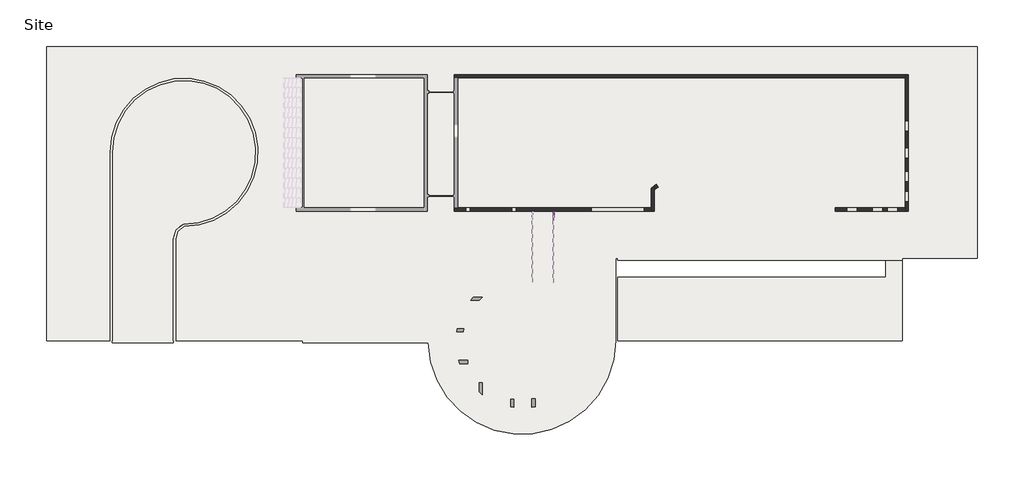
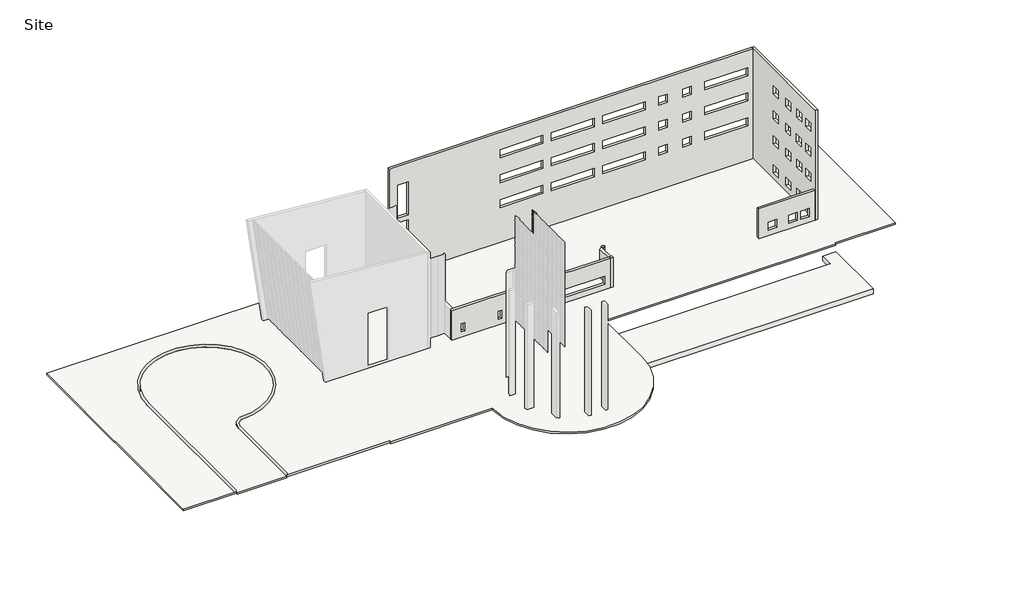
# One storey, part 4 of 4: 17 members, 6 walls, 3 slabs, 1 plate.
"""IFC4 building model written with IfcOpenShell, lengths in millimetres."""

import ifcopenshell
import ifcopenshell.guid

model = None  # the IFC model being written
_history = None  # IfcOwnerHistory: only IFC2X3 demands one
_inside = {}  # id of a spatial element -> (the spatial element, [elements in it])
_under = {}  # id of a project, library or spatial element -> (it, [spatial elements below it])
_declared = {}  # id of a project -> (the project, [libraries it declares])
_typed = {}  # id of a type object -> (the type object, [elements of that type])
_made_of = {}  # id of a material, layer set ... -> (it, [elements and type objects made of it])


def new_model(schema):
    """Start an empty IFC model of exactly this schema.

    Asked for "IFC4X3", IfcOpenShell would pick the latest addendum, in which some entities
    have other attributes; the version numbers below select the first issue.
    IFC2X3 requires an IfcOwnerHistory on every rooted entity: one is made here for all.
    """
    global model, _history
    if schema == "IFC4X3":
        model = ifcopenshell.file(schema_version=(4, 3, 0, 0))
    else:
        model = ifcopenshell.file(schema=schema)
    _inside.clear()
    _under.clear()
    _declared.clear()
    _typed.clear()
    _made_of.clear()
    _history = None
    if model.schema == "IFC2X3":
        org = make("IfcOrganization", Name="unknown")
        user = make(
            "IfcPersonAndOrganization",
            ThePerson=make("IfcPerson", FamilyName="unknown"),
            TheOrganization=org,
        )
        app = make(
            "IfcApplication",
            ApplicationDeveloper=org,
            Version="unknown",
            ApplicationFullName="unknown",
            ApplicationIdentifier="unknown",
        )
        _history = make(
            "IfcOwnerHistory",
            OwningUser=user,
            OwningApplication=app,
            ChangeAction="ADDED",
            CreationDate=0,
        )
    return model


def make(cls, **values):
    """One entity of the class cls with the attributes given. An attribute that is None is left unset."""
    return model.create_entity(
        cls, **{name: value for name, value in values.items() if value is not None}
    )


def rooted(cls, **values):
    """An entity with a GlobalId (a new one), such as an element, a storey or a relation."""
    return make(cls, GlobalId=ifcopenshell.guid.new(), OwnerHistory=_history, **values)


def si_unit(unit_type, name, prefix=None):
    """IfcSIUnit, for example si_unit("LENGTHUNIT", "METRE", prefix="MILLI")."""
    return make("IfcSIUnit", UnitType=unit_type, Prefix=prefix, Name=name)


def assignment(units):
    """IfcUnitAssignment: the units of a project."""
    return None if units is None else make("IfcUnitAssignment", Units=units)


def point(xyz):
    """IfcCartesianPoint."""
    return None if xyz is None else make("IfcCartesianPoint", Coordinates=xyz)


def direction(xyz):
    """IfcDirection."""
    return None if xyz is None else make("IfcDirection", DirectionRatios=xyz)


def frame(location, z_axis=None, x_axis=None):
    """IfcAxis2Placement3D, a coordinate frame: its origin and axes. An axis left out is left unset."""
    return make(
        "IfcAxis2Placement3D",
        Location=point(location),
        Axis=direction(z_axis),
        RefDirection=direction(x_axis),
    )


def frame_2d(location, x_axis=None):
    """IfcAxis2Placement2D, a coordinate frame in the plane: its origin and x axis."""
    return make(
        "IfcAxis2Placement2D", Location=point(location), RefDirection=direction(x_axis)
    )


def origin():
    """The frame at (0, 0, 0) with its axes left unset."""
    return frame((0.0, 0.0, 0.0))


def origin_with_axes():
    """The frame at (0, 0, 0) with the z axis (0, 0, 1) and the x axis (1, 0, 0) written out."""
    return frame((0.0, 0.0, 0.0), z_axis=(0.0, 0.0, 1.0), x_axis=(1.0, 0.0, 0.0))


def place(relative_to, where):
    """IfcLocalPlacement: puts the frame where relative to a parent placement (None: the world)."""
    return make(
        "IfcLocalPlacement", PlacementRelTo=relative_to, RelativePlacement=where
    )


def context(
    kind, dimensions, precision=None, world=None, true_north=None, identifier=None
):
    """IfcGeometricRepresentationContext, for example the 3D "Model" context."""
    return make(
        "IfcGeometricRepresentationContext",
        ContextIdentifier=identifier,
        ContextType=kind,
        CoordinateSpaceDimension=dimensions,
        Precision=precision,
        WorldCoordinateSystem=world,
        TrueNorth=true_north,
    )


def project(units=None, contexts=None):
    """IfcProject with its units and contexts."""
    return rooted(
        "IfcProject",
        Name="project",
        RepresentationContexts=contexts,
        UnitsInContext=assignment(units),
    )


def spatial(cls, under=None, at=None, **own):
    """A site, building, storey or space (cls), placed at a placement, below another one or the project."""
    s = rooted(cls, ObjectPlacement=at, **own)
    if under is not None:
        _under.setdefault(under.id(), (under, []))[1].append(s)
    return s


def polyline(points):
    """IfcPolyline through the points."""
    return make("IfcPolyline", Points=[point(p) for p in points])


def circle_curve(where, radius):
    """IfcCircle in the frame where."""
    return make("IfcCircle", Position=where, Radius=radius)


def trimmed(basis, trim1, trim2, sense, master):
    """IfcTrimmedCurve: the piece of a basis curve between two trims."""
    return make(
        "IfcTrimmedCurve",
        BasisCurve=basis,
        Trim1=trim1,
        Trim2=trim2,
        SenseAgreement=sense,
        MasterRepresentation=master,
    )


def segment(curve, same_sense, transition):
    """IfcCompositeCurveSegment."""
    return make(
        "IfcCompositeCurveSegment",
        Transition=transition,
        SameSense=same_sense,
        ParentCurve=curve,
    )


def composite_curve(segments, self_intersect=None):
    """IfcCompositeCurve: segments joined end to end."""
    return make("IfcCompositeCurve", Segments=segments, SelfIntersect=self_intersect)


def outline(outer, holes=None, kind="AREA"):
    """IfcArbitraryClosedProfileDef: a profile drawn as a closed curve; with holes, ...WithVoids."""
    if holes is None:
        return make("IfcArbitraryClosedProfileDef", ProfileType=kind, OuterCurve=outer)
    return make(
        "IfcArbitraryProfileDefWithVoids",
        ProfileType=kind,
        OuterCurve=outer,
        InnerCurves=holes,
    )


def extrude(swept, where, along, depth):
    """IfcExtrudedAreaSolid: the profile swept, set in the frame where, extruded along a direction by depth."""
    return make(
        "IfcExtrudedAreaSolid",
        SweptArea=swept,
        Position=where,
        ExtrudedDirection=direction(along),
        Depth=depth,
    )


def faces_of(points, faces, orient=None, outer=None):
    """IfcFace entities. A face is a list of loops; a loop is a list of indices into points, from 0.

    orient and outer hold one flag for each loop. By default every Orientation is true, the
    first loop of a face is its IfcFaceOuterBound and the others are IfcFaceBound.
    """
    made = []
    for i, loops in enumerate(faces):
        bounds = []
        for j, loop in enumerate(loops):
            is_outer = j == 0 if outer is None else outer[i][j]
            bounds.append(
                make(
                    "IfcFaceOuterBound" if is_outer else "IfcFaceBound",
                    Bound=make("IfcPolyLoop", Polygon=[points[k] for k in loop]),
                    Orientation=True if orient is None else orient[i][j],
                )
            )
        made.append(make("IfcFace", Bounds=bounds))
    return made


def faceted_brep(points, faces, orient=None, outer=None, voids=None):
    """IfcFacetedBrep: a solid bounded by flat faces; with voids (closed shells), ...WithVoids."""
    shared = [point(p) for p in points]
    hull = make("IfcClosedShell", CfsFaces=faces_of(shared, faces, orient, outer))
    if voids is None:
        return make("IfcFacetedBrep", Outer=hull)
    return make(
        "IfcFacetedBrepWithVoids",
        Outer=hull,
        Voids=[
            make(cls, CfsFaces=faces_of(shared, fs, o, b)) for cls, fs, o, b in voids
        ],
    )


def shape(context_of_items, identifier, shape_type, items):
    """IfcShapeRepresentation: the items that make up one representation, for example the "Body"."""
    return make(
        "IfcShapeRepresentation",
        ContextOfItems=context_of_items,
        RepresentationIdentifier=identifier,
        RepresentationType=shape_type,
        Items=items,
    )


def source(mapping_origin, context_of_items, identifier, shape_type, items):
    """IfcRepresentationMap: a shape defined once, which mapped items show again and again."""
    return make(
        "IfcRepresentationMap",
        MappingOrigin=mapping_origin,
        MappedRepresentation=shape(context_of_items, identifier, shape_type, items),
    )


def transform(
    local_origin,
    x_axis=None,
    y_axis=None,
    z_axis=None,
    scale=None,
    scale2=None,
    scale3=None,
    uniform=True,
):
    """IfcCartesianTransformationOperator3D, or its non-uniform kind. x_axis, y_axis, z_axis: its Axis1, 2, 3."""
    if uniform:
        return make(
            "IfcCartesianTransformationOperator3D",
            Axis1=direction(x_axis),
            Axis2=direction(y_axis),
            LocalOrigin=point(local_origin),
            Scale=scale,
            Axis3=direction(z_axis),
        )
    return make(
        "IfcCartesianTransformationOperator3DnonUniform",
        Axis1=direction(x_axis),
        Axis2=direction(y_axis),
        LocalOrigin=point(local_origin),
        Scale=scale,
        Axis3=direction(z_axis),
        Scale2=scale2,
        Scale3=scale3,
    )


def mapped(mapping_source, mapping_target):
    """IfcMappedItem: shows the shape of a source again, moved by a transform."""
    return make(
        "IfcMappedItem", MappingSource=mapping_source, MappingTarget=mapping_target
    )


def made_of(thing, what):
    """Note that an element or type object is made of a material, layer set ...; save() writes the relation."""
    if what is not None:
        _made_of.setdefault(what.id(), (what, []))[1].append(thing)
    return thing


def element(
    cls,
    number,
    at=None,
    inside=None,
    cuts=None,
    type_object=None,
    material=None,
    context=None,
    identifier="Body",
    shape_type=None,
    held_by="IfcProductDefinitionShape",
    body=None,
    shapes=None,
    **own,
):
    """One element of the class cls, such as IfcWall. Its Tag is "e" and its number.

    at: its placement. inside: the storey or other place that contains it. cuts: it is an
    opening in that element (IfcRelVoidsElement). A single representation is given by context,
    identifier, shape_type and body (its items); several are given by shapes. held_by: the class
    of the entity that holds the representations. save() writes the other relations.
    """
    e = rooted(cls, Tag="e%d" % number, ObjectPlacement=at, **own)
    if body is not None:
        shapes = [shape(context, identifier, shape_type, body)]
    if shapes is not None:
        e.Representation = make(held_by, Representations=shapes)
    if inside is not None:
        _inside.setdefault(inside.id(), (inside, []))[1].append(e)
    if cuts is not None:
        rooted(
            "IfcRelVoidsElement", RelatingBuildingElement=cuts, RelatedOpeningElement=e
        )
    if type_object is not None:
        _typed.setdefault(type_object.id(), (type_object, []))[1].append(e)
    return made_of(e, material)


def aggregate(whole, parts):
    """IfcRelAggregates: a whole, such as a stair, and the parts it consists of."""
    return rooted("IfcRelAggregates", RelatingObject=whole, RelatedObjects=parts)


def save(model, path):
    """Write the relations noted so far, then the file.

    IfcRelAggregates (storeys below a building ...), IfcRelContainedInSpatialStructure (elements
    in a storey), IfcRelDefinesByType, IfcRelAssociatesMaterial and IfcRelDeclares: one each for
    every whole, place, type object, material and project.
    """
    for whole, parts in _under.values():
        aggregate(whole, parts)
    for where, things in _inside.values():
        rooted(
            "IfcRelContainedInSpatialStructure",
            RelatedElements=things,
            RelatingStructure=where,
        )
    for kind, things in _typed.values():
        rooted("IfcRelDefinesByType", RelatedObjects=things, RelatingType=kind)
    for what, things in _made_of.values():
        rooted("IfcRelAssociatesMaterial", RelatedObjects=things, RelatingMaterial=what)
    for by, libraries in _declared.values():
        rooted("IfcRelDeclares", RelatingContext=by, RelatedDefinitions=libraries)
    model.write(path)


def plane_surface(at):
    """IfcPlane: the flat surface through the origin of the frame at, square to its z axis."""
    return make("IfcPlane", Position=at)


def cylinder_surface(at, radius):
    """IfcCylindricalSurface: all points at the distance radius from the z axis of the frame at."""
    return make("IfcCylindricalSurface", Position=at, Radius=radius)


def revolved_surface(curve, axis_point, axis_direction):
    """IfcSurfaceOfRevolution: the curve turned about the line through axis_point along axis_direction."""
    return make(
        "IfcSurfaceOfRevolution",
        SweptCurve=make("IfcArbitraryOpenProfileDef", ProfileType="CURVE", Curve=curve),
        AxisPosition=make("IfcAxis1Placement", Location=point(axis_point), Axis=direction(axis_direction)),
    )


def advanced_brep(points, edges, surfaces, faces):
    """IfcAdvancedBrep: a solid bounded by faces that lie on surfaces and meet in shared edges.

    An edge is (start, end): straight between two places in points (the first is 0);
    or (start, end, curve); or (start, end, curve, False) where it runs against its curve.
    A face is (place in surfaces, loops), or (place, loops, False) where it looks against
    its surface's normal. A loop lists edges by number (the first is 1), with a minus sign
    where the edge is run from its end to its start. The first loop is the outer one.
    """
    corners = [point(p) for p in points]
    vertices = [make("IfcVertexPoint", VertexGeometry=c) for c in corners]
    made = []
    for start, end, *more in edges:
        made.append(
            make(
                "IfcEdgeCurve",
                EdgeStart=vertices[start],
                EdgeEnd=vertices[end],
                EdgeGeometry=more[0] if more else make("IfcPolyline", Points=[corners[start], corners[end]]),
                SameSense=more[1] if len(more) > 1 else True,
            )
        )
    hull = []
    for where, loops, *sense in faces:
        bounds = []
        for j, loop in enumerate(loops):
            ring = [make("IfcOrientedEdge", EdgeElement=made[abs(k) - 1], Orientation=k > 0) for k in loop]
            bounds.append(
                make(
                    "IfcFaceOuterBound" if j == 0 else "IfcFaceBound",
                    Bound=make("IfcEdgeLoop", EdgeList=ring),
                    Orientation=True,
                )
            )
        hull.append(make("IfcAdvancedFace", Bounds=bounds, FaceSurface=surfaces[where], SameSense=sense[0] if sense else True))
    return make("IfcAdvancedBrep", Outer=make("IfcClosedShell", CfsFaces=hull))


def member_5d07894b(model_context):
    return source(origin(), model_context, "Body", "SweptSolid", [
        extrude(outline(polyline([(31.75, 63.5), (31.75, -63.5), (-31.75, -63.5), (-31.75, 63.5), (31.75, 63.5)])), frame((0.0, 0.0, -4629.15), z_axis=(0.0, 0.0, 1.0), x_axis=(1.0, 0.0, 0.0)), (0.0, 0.0, 1.0), 4629.15),
    ])


def member_3ba9e939(model_context):
    return source(origin(), model_context, "Body", "SweptSolid", [
        extrude(outline(polyline([(31.75, 63.5), (31.75, -63.5), (-31.75, -63.5), (-31.75, 63.5), (31.75, 63.5)])), frame((0.0, 0.0, -3746.5), z_axis=(0.0, 0.0, 1.0), x_axis=(1.0, 0.0, 0.0)), (0.0, 0.0, 1.0), 3746.5),
    ])


def member_ad567e07(model_context):
    return source(origin(), model_context, "Body", "SweptSolid", [
        extrude(outline(polyline([(31.75, 63.5), (31.75, -63.5), (-31.75, -63.5), (-31.75, 63.5), (31.75, 63.5)])), frame((0.0, 0.0, -819.15), z_axis=(0.0, 0.0, 1.0), x_axis=(1.0, 0.0, 0.0)), (0.0, 0.0, 1.0), 819.15),
    ])


def member_7db1855a(model_context):
    return source(origin(), model_context, "Body", "SweptSolid", [
        extrude(outline(polyline([(31.75, 63.5), (31.75, -63.5), (-31.75, -63.5), (-31.75, 63.5), (31.75, 63.5)])), frame((0.0, 0.0, -850.9), z_axis=(0.0, 0.0, 1.0), x_axis=(1.0, 0.0, 0.0)), (0.0, 0.0, 1.0), 850.9),
    ])


def member_ffd4c858(model_context):
    return source(origin(), model_context, "Body", "SweptSolid", [
        extrude(outline(polyline([(31.75, 63.5), (31.75, -63.5), (-31.75, -63.5), (-31.75, 63.5), (31.75, 63.5)])), frame((0.0, 0.0, -457.2), z_axis=(0.0, 0.0, 1.0), x_axis=(1.0, 0.0, 0.0)), (0.0, 0.0, 1.0), 457.2),
    ])


def member_15823cb3(model_context):
    return source(origin(), model_context, "Body", "SweptSolid", [
        extrude(outline(polyline([(0.0, 63.5), (0.0, -63.5), (-63.5, -63.5), (-63.5, 63.5), (0.0, 63.5)])), frame((0.0, 0.0, -457.2), z_axis=(0.0, 0.0, 1.0), x_axis=(1.0, 0.0, 0.0)), (0.0, 0.0, 1.0), 457.2),
    ])


def member_e9605c56(model_context):
    return source(origin(), model_context, "Body", "SweptSolid", [
        extrude(outline(polyline([(0.0, 63.5), (0.0, -63.5), (-63.5, -63.5), (-63.5, 63.5), (0.0, 63.5)])), frame((0.0, 0.0, -825.5), z_axis=(0.0, 0.0, 1.0), x_axis=(1.0, 0.0, 0.0)), (0.0, 0.0, 1.0), 825.5),
    ])


def system_panel_glazed_cc98a0ec(model_context):
    return source(origin(), model_context, "Body", "SweptSolid", [
        extrude(outline(polyline([(180.975, 19.05), (-180.975, 19.05), (-180.975, 44.45), (180.975, 44.45), (180.975, 19.05)])), origin_with_axes(), (0.0, 0.0, 1.0), 819.15),
    ])


model = new_model("IFC4")

# Units and contexts
model_context = context("Model", 3, world=origin())
ifc_project = project(units=[si_unit("LENGTHUNIT", "METRE", prefix="MILLI")], contexts=[model_context])

# Site, building, storey
site = spatial("IfcSite", under=ifc_project)
building = spatial("IfcBuilding", under=site)
storey = spatial("IfcBuildingStorey", under=building, Name="Site", Elevation=-152.4)

# Members
placement = place(None, origin())
member_shape = member_5d07894b(model_context)
element("IfcMember", 1, ObjectType="Rectangular Mullion1 : 2.5\" x 5\" rectangular", at=placement, inside=storey, context=model_context, shape_type="MappedRepresentation", body=[
    mapped(member_shape, transform((10878.8276119, 37629.311889, -88.9), x_axis=(0.0, 1.0, 0.0), y_axis=(1.0, 0.0, 0.0), z_axis=(0.0, 0.0, -1.0))),
])
member_2_shape = member_3ba9e939(model_context)
element("IfcMember", 2, ObjectType="Rectangular Mullion1 : 2.5\" x 5\" rectangular", at=placement, inside=storey, context=model_context, shape_type="MappedRepresentation", body=[
    mapped(member_2_shape, transform((10878.8276119, 37629.311889, 5518.15), x_axis=(0.0, 1.0, 0.0), y_axis=(1.0, 0.0, 0.0), z_axis=(0.0, 0.0, -1.0))),
])
element("IfcMember", 3, ObjectType="Rectangular Mullion1 : 2.5\" x 5\" rectangular", at=placement, inside=storey, context=model_context, shape_type="MappedRepresentation", body=[
    mapped(member_2_shape, transform((10878.8276119, 37629.311889, 10242.55), x_axis=(0.0, 1.0, 0.0), y_axis=(1.0, 0.0, 0.0), z_axis=(0.0, 0.0, -1.0))),
])
element("IfcMember", 4, ObjectType="Rectangular Mullion1 : 2.5\" x 5\" rectangular", at=placement, inside=storey, context=model_context, shape_type="MappedRepresentation", body=[
    mapped(member_2_shape, transform((10878.8276119, 37629.311889, 14966.95), x_axis=(0.0, 1.0, 0.0), y_axis=(1.0, 0.0, 0.0), z_axis=(0.0, 0.0, -1.0))),
])
member_3_shape = member_ad567e07(model_context)
element("IfcMember", 5, ObjectType="Rectangular Mullion1 : 2.5\" x 5\" rectangular", at=placement, inside=storey, context=model_context, shape_type="MappedRepresentation", body=[
    mapped(member_3_shape, transform((10878.8276119, 37629.311889, 18776.95), x_axis=(0.0, 1.0, 0.0), y_axis=(1.0, 0.0, 0.0), z_axis=(0.0, 0.0, -1.0))),
])
member_4_shape = member_7db1855a(model_context)
element("IfcMember", 6, ObjectType="Rectangular Mullion1 : 2.5\" x 5\" rectangular", at=placement, inside=storey, context=model_context, shape_type="MappedRepresentation", body=[
    mapped(member_4_shape, transform((10878.8276119, 37629.311889, 14052.55), x_axis=(0.0, 1.0, 0.0), y_axis=(1.0, 0.0, 0.0), z_axis=(0.0, 0.0, -1.0))),
])
element("IfcMember", 7, ObjectType="Rectangular Mullion1 : 2.5\" x 5\" rectangular", at=placement, inside=storey, context=model_context, shape_type="MappedRepresentation", body=[
    mapped(member_4_shape, transform((10878.8276119, 37629.311889, 4603.75), x_axis=(0.0, 1.0, 0.0), y_axis=(1.0, 0.0, 0.0), z_axis=(0.0, 0.0, -1.0))),
])
element("IfcMember", 8, ObjectType="Rectangular Mullion1 : 2.5\" x 5\" rectangular", at=placement, inside=storey, context=model_context, shape_type="MappedRepresentation", body=[
    mapped(member_4_shape, transform((10878.8276119, 37629.311889, 9328.15), x_axis=(0.0, 1.0, 0.0), y_axis=(1.0, 0.0, 0.0), z_axis=(0.0, 0.0, -1.0))),
])
member_5_shape = member_ffd4c858(model_context)
element("IfcMember", 9, ObjectType="Rectangular Mullion1 : 2.5\" x 5\" rectangular", at=placement, inside=storey, context=model_context, shape_type="MappedRepresentation", body=[
    mapped(member_5_shape, transform((10878.8276119, 38086.511889, 14935.2), x_axis=(0.0, 0.0, 1.0), y_axis=(1.0, 0.0, 0.0), z_axis=(0.0, 1.0, 0.0))),
])
element("IfcMember", 10, ObjectType="Rectangular Mullion1 : 2.5\" x 5\" rectangular", at=placement, inside=storey, context=model_context, shape_type="MappedRepresentation", body=[
    mapped(member_5_shape, transform((10878.8276119, 38086.511889, 10210.8), x_axis=(0.0, 0.0, 1.0), y_axis=(1.0, 0.0, 0.0), z_axis=(0.0, 1.0, 0.0))),
])
element("IfcMember", 11, ObjectType="Rectangular Mullion1 : 2.5\" x 5\" rectangular", at=placement, inside=storey, context=model_context, shape_type="MappedRepresentation", body=[
    mapped(member_5_shape, transform((10878.8276119, 38086.511889, 5486.4), x_axis=(0.0, 0.0, 1.0), y_axis=(1.0, 0.0, 0.0), z_axis=(0.0, 1.0, 0.0))),
])
element("IfcMember", 12, ObjectType="Rectangular Mullion1 : 2.5\" x 5\" rectangular", at=placement, inside=storey, context=model_context, shape_type="MappedRepresentation", body=[
    mapped(member_5_shape, transform((10878.8276119, 38086.511889, 9296.4), x_axis=(0.0, 0.0, 1.0), y_axis=(1.0, 0.0, 0.0), z_axis=(0.0, 1.0, 0.0))),
])
element("IfcMember", 13, ObjectType="Rectangular Mullion1 : 2.5\" x 5\" rectangular", at=placement, inside=storey, context=model_context, shape_type="MappedRepresentation", body=[
    mapped(member_5_shape, transform((10878.8276119, 38086.511889, 4572.0), x_axis=(0.0, 0.0, 1.0), y_axis=(1.0, 0.0, 0.0), z_axis=(0.0, 1.0, 0.0))),
])
element("IfcMember", 14, ObjectType="Rectangular Mullion1 : 2.5\" x 5\" rectangular", at=placement, inside=storey, context=model_context, shape_type="MappedRepresentation", body=[
    mapped(member_5_shape, transform((10878.8276119, 38086.511889, 14020.8), x_axis=(0.0, 0.0, 1.0), y_axis=(1.0, 0.0, 0.0), z_axis=(0.0, 1.0, 0.0))),
])
element("IfcMember", 15, ObjectType="Rectangular Mullion1 : 2.5\" x 5\" rectangular", at=placement, inside=storey, context=model_context, shape_type="MappedRepresentation", body=[
    mapped(member_5_shape, transform((10878.8276119, 38086.511889, 18745.2), x_axis=(0.0, 0.0, 1.0), y_axis=(1.0, 0.0, 0.0), z_axis=(0.0, 1.0, 0.0))),
])
member_6_shape = member_15823cb3(model_context)
element("IfcMember", 16, ObjectType="Rectangular Mullion1 : 2.5\" x 5\" rectangular", at=placement, inside=storey, context=model_context, shape_type="MappedRepresentation", body=[
    mapped(member_6_shape, transform((10878.8276119, 37629.311889, -152.4), x_axis=(0.0, 0.0, -1.0), y_axis=(1.0, 0.0, 0.0), z_axis=(0.0, -1.0, 0.0))),
])
member_7_shape = member_e9605c56(model_context)
element("IfcMember", 17, ObjectType="Rectangular Mullion1 : 2.5\" x 5\" rectangular", at=placement, inside=storey, context=model_context, shape_type="MappedRepresentation", body=[
    mapped(member_7_shape, transform((10878.8276119, 37629.311889, 19659.6), x_axis=(0.0, 0.0, 1.0), y_axis=(1.0, 0.0, 0.0), z_axis=(0.0, 1.0, 0.0))),
])

# Plate
system_panel_glazed_shape = system_panel_glazed_cc98a0ec(model_context)
element("IfcPlate", 18, ObjectType="System Panel : Glazed", at=placement, inside=storey, context=model_context, shape_type="MappedRepresentation", body=[
    mapped(system_panel_glazed_shape, transform((10878.8276119, 37842.036889, 18776.95), x_axis=(0.0, 1.0, 0.0), y_axis=(-1.0, 0.0, 0.0), z_axis=(0.0, 0.0, 1.0))),
])

# Slabs
element("IfcSlab", 19, ObjectType="a_drive", at=placement, inside=storey, context=model_context, shape_type="SweptSolid", body=[
    extrude(outline(composite_curve([segment(trimmed(circle_curve(frame_2d((-42359.2307976, 46620.911889)), 10363.2), [point((-52722.4307976, 46620.911889))], [point((-42384.6461103, 36257.743054))], False, "CARTESIAN"), True, "CONTINUOUS"), segment(trimmed(circle_curve(frame_2d((-41679.1721267, 34169.1174245)), 2204.5522361), [point((-42384.6461103, 36257.743054))], [point((-43883.2307976, 34122.4704857))], True, "CARTESIAN"), True, "CONTINUOUS"), segment(polyline([(-43883.2307976, 34122.4704857), (-43883.2307976, 19188.911889), (-52722.4307976, 19188.911889), (-52722.4307976, 46620.911889)]), True, "CONTINUOUS")], self_intersect=False)), frame((0.0, 0.0, -457.2), z_axis=(0.0, 0.0, 1.0), x_axis=(1.0, 0.0, 0.0)), (0.0, 0.0, 1.0), 304.8),
])
element("IfcSlab", 20, ObjectType="a_site paving", at=placement, inside=storey, context=model_context, shape_type="SweptSolid", body=[
    extrude(outline(composite_curve([segment(polyline([(71940.7692024, 61860.911889), (71940.7692024, 31380.911889), (61120.3692024, 31380.911889), (61120.3692024, 31076.111889), (20124.7692024, 31076.111889), (20124.7692024, 31380.911889), (19819.9692024, 31380.911889), (19819.9692024, 19493.711889)]), True, "CONTINUOUS"), segment(trimmed(circle_curve(frame_2d((6332.9997246, 19493.711889)), 13486.9694778), [point((19819.9692024, 19493.711889))], [point((-7150.5251356, 19188.911889))], False, "CARTESIAN"), True, "CONTINUOUS"), segment(polyline([(-7150.5251356, 19188.911889), (-25290.4307976, 19188.911889), (-25290.4307976, 19493.711889), (-43883.2307976, 19493.711889), (-43883.2307976, 34122.4704857)]), True, "CONTINUOUS"), segment(trimmed(circle_curve(frame_2d((-41679.1721267, 34169.1174245)), 2204.5522361), [point((-43883.2307976, 34122.4704857))], [point((-42384.6461103, 36257.743054))], False, "CARTESIAN"), True, "CONTINUOUS"), segment(trimmed(circle_curve(frame_2d((-42359.2307976, 46620.911889)), 10363.2), [point((-42384.6461103, 36257.743054))], [point((-52722.4307976, 46620.911889))], True, "CARTESIAN"), True, "CONTINUOUS"), segment(polyline([(-52722.4307976, 46620.911889), (-52722.4307976, 19493.711889), (-62171.2307976, 19493.711889), (-62171.2307976, 61860.911889), (71940.7692024, 61860.911889)]), True, "CONTINUOUS")], self_intersect=False)), frame((0.0, 0.0, -457.2), z_axis=(0.0, 0.0, 1.0), x_axis=(1.0, 0.0, 0.0)), (0.0, 0.0, 1.0), 304.8),
])
element("IfcSlab", 21, ObjectType="water feature", at=placement, inside=storey, context=model_context, shape_type="SweptSolid", body=[
    extrude(outline(polyline([(20124.7692024, 28656.761889), (58732.7692024, 28656.761889), (58732.7692024, 31076.111889), (61120.3692024, 31076.111889), (61120.3692024, 19493.711889), (20124.7692024, 19493.711889), (20124.7692024, 28656.761889)])), frame((0.0, 0.0, -2590.8), z_axis=(0.0, 0.0, 1.0), x_axis=(1.0, 0.0, 0.0)), (0.0, 0.0, 1.0), 914.4),
])

# Walls
element("IfcWall", 22, ObjectType="Stone on CMU", at=placement, inside=storey, context=model_context, shape_type="AdvancedBrep", body=[
    advanced_brep(
    [(24926.9567024, 41466.5312272, -152.4), (24926.9567024, 38618.324389, -152.4), (24926.9567024, 38164.299389, -152.4), (24926.9567024, 38164.299389, 5486.4), (24926.9567024, 38618.324389, 5486.4), (24926.9567024, 38618.324389, 5181.6), (24926.9567024, 41466.5312272, 5181.6), (25380.9817024, 41789.4772012, -152.4), (25380.9817024, 41789.4772012, 5181.6), (25380.9817024, 38618.324389, 5181.6), (25380.9817024, 38618.324389, 5486.4), (25380.9817024, 38164.299389, 5486.4), (25380.9817024, 38164.299389, -152.4), (25380.9817024, 41234.3316602, -152.4)],
    [
        (0, 1),
        (1, 2),
        (2, 3),
        (3, 4),
        (4, 5),
        (5, 6),
        (6, 0),
        (7, 8),
        (8, 9),
        (9, 10),
        (10, 11),
        (11, 12),
        (12, 13),
        (13, 7),
        (0, 7, circle_curve(frame((38486.136956, 22884.5054507, -152.4), z_axis=(0.0, 0.0, -1.0), x_axis=(1.0, 0.0, 0.0)), 23003.1095965)),
        (12, 2),
        (3, 11),
        (10, 4),
        (9, 5),
        (8, 6, circle_curve(frame((38486.136956, 22884.5054507, 5181.6), z_axis=(0.0, 0.0, 1.0), x_axis=(1.0, 0.0, 0.0)), 23003.1095965)),
    ],
    [
        plane_surface(frame((24926.9567024, 41350.796414, -152.4), z_axis=(-1.0, 0.0, 0.0), x_axis=(0.0, -1.0, 0.0))),
        plane_surface(frame((25380.9817024, 41350.796414, -152.4), z_axis=(1.0, 0.0, 0.0), x_axis=(0.0, 1.0, 0.0))),
        plane_surface(frame((24926.9567024, 41350.796414, -152.4), z_axis=(0.0, 0.0, -1.0), x_axis=(1.0, 0.0, 0.0))),
        plane_surface(frame((24926.9567024, 38391.311889, 5486.4), z_axis=(0.0, 0.0, 1.0), x_axis=(1.0, 0.0, 0.0))),
        plane_surface(frame((24926.9567024, 38618.324389, 5486.4), z_axis=(0.0, 1.0, 0.0), x_axis=(1.0, 0.0, 0.0))),
        plane_surface(frame((24926.9567024, 38618.324389, 5181.6), z_axis=(0.0, 0.0, 1.0), x_axis=(1.0, 0.0, 0.0))),
        plane_surface(frame((24696.7692024, 38164.299389, -152.4), z_axis=(0.0, -1.0, 0.0), x_axis=(1.0, 0.0, 0.0))),
        cylinder_surface(frame((38486.136956, 22884.5054507, -152.4), z_axis=(0.0, 0.0, 1.0), x_axis=(1.0, 0.0, 0.0)), 23003.1095965),
    ],
    [
        (0, [[1, 2, 3, 4, 5, 6, 7]]),
        (1, [[8, 9, 10, 11, 12, 13, 14]]),
        (2, [[-2, -1, 15, -14, -13, 16]]),
        (3, [[-4, 17, -11, 18]]),
        (4, [[-5, -18, -10, 19]]),
        (5, [[-6, -19, -9, 20]]),
        (6, [[-3, -16, -12, -17]]),
        (7, [[-7, -20, -8, -15]]),
    ],
),
])
element("IfcWall", 23, ObjectType="Stone on CMU", at=placement, inside=storey, context=model_context, shape_type="Brep", body=[
    faceted_brep([(24926.9567024, 38618.324389, 5486.4), (6799.2942024, 38618.324389, 5486.4), (6656.4192024, 38618.324389, 5486.4), (-2965.7977165, 38618.324389, 5486.4), (-3419.8227165, 38618.324389, 5486.4), (-3419.8227165, 38164.299389, 5486.4), (24926.9567024, 38164.299389, 5486.4), (24926.9567024, 38618.324389, -152.4), (-2965.7977165, 38618.324389, -152.4), (-3419.8227165, 38618.324389, -152.4), (24926.9567024, 38618.324389, 5181.6), (4884.7692024, 38618.324389, 2438.4), (4884.7692024, 38618.324389, 914.4), (5494.3692024, 38618.324389, 914.4), (5494.3692024, 38618.324389, 2438.4), (-1750.9807976, 38618.324389, 2438.4), (-1750.9807976, 38618.324389, 914.4), (-1141.3807976, 38618.324389, 914.4), (-1141.3807976, 38618.324389, 2438.4), (16314.7692024, 38618.324389, 2438.4), (16314.7692024, 38618.324389, 914.4), (23934.7692024, 38618.324389, 914.4), (23934.7692024, 38618.324389, 2438.4), (24926.9567024, 38164.299389, -152.4), (-3419.8227165, 38164.299389, -152.4), (4884.7692024, 38164.299389, 2438.4), (5494.3692024, 38164.299389, 2438.4), (5494.3692024, 38164.299389, 914.4), (4884.7692024, 38164.299389, 914.4), (-1750.9807976, 38164.299389, 2438.4), (-1141.3807976, 38164.299389, 2438.4), (-1141.3807976, 38164.299389, 914.4), (-1750.9807976, 38164.299389, 914.4), (16314.7692024, 38164.299389, 2438.4), (23934.7692024, 38164.299389, 2438.4), (23934.7692024, 38164.299389, 914.4), (16314.7692024, 38164.299389, 914.4)], [[[0, 1, 2, 3, 4, 5, 6]], [[7, 8, 9, 4, 3, 2, 1, 0, 10], [11, 12, 13, 14], [15, 16, 17, 18], [19, 20, 21, 22]], [[23, 6, 5, 24], [25, 26, 27, 28], [29, 30, 31, 32], [33, 34, 35, 36]], [[9, 8, 7, 23, 24]], [[7, 10, 0, 6, 23]], [[4, 9, 24, 5]], [[12, 11, 25, 28]], [[13, 12, 28, 27]], [[14, 13, 27, 26]], [[11, 14, 26, 25]], [[16, 15, 29, 32]], [[17, 16, 32, 31]], [[18, 17, 31, 30]], [[15, 18, 30, 29]], [[20, 19, 33, 36]], [[21, 20, 36, 35]], [[22, 21, 35, 34]], [[19, 22, 34, 33]]]),
])
element("IfcWall", 24, ObjectType="Stone on CMU", at=placement, inside=storey, context=model_context, shape_type="Brep", body=[
    faceted_brep([(61502.9567024, 38618.324389, -152.4), (51444.5567024, 38618.324389, -152.4), (51444.5567024, 38618.324389, 0.0), (51444.5567024, 38618.324389, 5181.6), (51444.5567024, 38618.324389, 5486.4), (61502.9567024, 38618.324389, 5486.4), (53119.3692024, 38618.324389, 2438.4), (53119.3692024, 38618.324389, 914.4), (54643.3692024, 38618.324389, 914.4), (54643.3692024, 38618.324389, 2438.4), (56776.9692024, 38618.324389, 2438.4), (56776.9692024, 38618.324389, 914.4), (58300.9692024, 38618.324389, 914.4), (58300.9692024, 38618.324389, 2438.4), (58910.5692024, 38618.324389, 2438.4), (58910.5692024, 38618.324389, 914.4), (60434.5692024, 38618.324389, 914.4), (60434.5692024, 38618.324389, 2438.4), (61502.9567024, 38164.299389, -152.4), (61502.9567024, 38164.299389, 5486.4), (51444.5567024, 38164.299389, 5486.4), (51444.5567024, 38164.299389, -152.4), (53119.3692024, 38164.299389, 2438.4), (54643.3692024, 38164.299389, 2438.4), (54643.3692024, 38164.299389, 914.4), (53119.3692024, 38164.299389, 914.4), (56776.9692024, 38164.299389, 2438.4), (58300.9692024, 38164.299389, 2438.4), (58300.9692024, 38164.299389, 914.4), (56776.9692024, 38164.299389, 914.4), (58910.5692024, 38164.299389, 2438.4), (60434.5692024, 38164.299389, 2438.4), (60434.5692024, 38164.299389, 914.4), (58910.5692024, 38164.299389, 914.4)], [[[0, 1, 2, 3, 4, 5], [6, 7, 8, 9], [10, 11, 12, 13], [14, 15, 16, 17]], [[18, 19, 20, 21], [22, 23, 24, 25], [26, 27, 28, 29], [30, 31, 32, 33]], [[1, 0, 18, 21]], [[5, 4, 20, 19]], [[4, 3, 2, 1, 21, 20]], [[0, 5, 19, 18]], [[7, 6, 22, 25]], [[8, 7, 25, 24]], [[9, 8, 24, 23]], [[6, 9, 23, 22]], [[11, 10, 26, 29]], [[12, 11, 29, 28]], [[13, 12, 28, 27]], [[10, 13, 27, 26]], [[15, 14, 30, 33]], [[16, 15, 33, 32]], [[17, 16, 32, 31]], [[14, 17, 31, 30]]]),
])
element("IfcWall", 25, ObjectType="Stone on CMU", at=placement, inside=storey, context=model_context, shape_type="Brep", body=[
    faceted_brep([(-3419.8227165, 57366.699389, -152.4), (-2965.7977165, 57366.699389, -152.4), (61502.9567024, 57366.699389, -152.4), (61502.9567024, 57366.699389, 20574.0), (-2965.7977165, 57366.699389, 20574.0), (-3419.8227165, 57366.699389, 20574.0), (-3419.8227165, 57366.699389, 5486.4), (-1998.6307976, 57366.699389, 10820.4), (-1998.6307976, 57366.699389, 17068.8), (-169.8307976, 57366.699389, 17068.8), (-169.8307976, 57366.699389, 10820.4), (-1998.6307976, 57366.699389, 3657.6), (-1998.6307976, 57366.699389, 9906.0), (-169.8307976, 57366.699389, 9906.0), (-169.8307976, 57366.699389, 3657.6), (50452.3692024, 57366.699389, 17373.6), (50452.3692024, 57366.699389, 15849.6), (48928.3692024, 57366.699389, 15849.6), (48928.3692024, 57366.699389, 17373.6), (46185.1692024, 57366.699389, 17373.6), (46185.1692024, 57366.699389, 15849.6), (44661.1692024, 57366.699389, 15849.6), (44661.1692024, 57366.699389, 17373.6), (50452.3692024, 57366.699389, 12649.2), (50452.3692024, 57366.699389, 11125.2), (48928.3692024, 57366.699389, 11125.2), (48928.3692024, 57366.699389, 12649.2), (46185.1692024, 57366.699389, 12649.2), (46185.1692024, 57366.699389, 11125.2), (44661.1692024, 57366.699389, 11125.2), (44661.1692024, 57366.699389, 12649.2), (50452.3692024, 57366.699389, 7924.8), (50452.3692024, 57366.699389, 6400.8), (48928.3692024, 57366.699389, 6400.8), (48928.3692024, 57366.699389, 7924.8), (46185.1692024, 57366.699389, 7924.8), (46185.1692024, 57366.699389, 6400.8), (44661.1692024, 57366.699389, 6400.8), (44661.1692024, 57366.699389, 7924.8), (60510.7692024, 57366.699389, 17373.6), (60510.7692024, 57366.699389, 15849.6), (52890.7692024, 57366.699389, 15849.6), (52890.7692024, 57366.699389, 17373.6), (60510.7692024, 57366.699389, 12649.2), (60510.7692024, 57366.699389, 11125.2), (52890.7692024, 57366.699389, 11125.2), (52890.7692024, 57366.699389, 12649.2), (60510.7692024, 57366.699389, 7924.8), (60510.7692024, 57366.699389, 6400.8), (52890.7692024, 57366.699389, 6400.8), (52890.7692024, 57366.699389, 7924.8), (23934.7692024, 57366.699389, 17373.6), (23934.7692024, 57366.699389, 15849.6), (16314.7692024, 57366.699389, 15849.6), (16314.7692024, 57366.699389, 17373.6), (23934.7692024, 57366.699389, 12649.2), (23934.7692024, 57366.699389, 11125.2), (16314.7692024, 57366.699389, 11125.2), (16314.7692024, 57366.699389, 12649.2), (23934.7692024, 57366.699389, 7924.8), (23934.7692024, 57366.699389, 6400.8), (16314.7692024, 57366.699389, 6400.8), (16314.7692024, 57366.699389, 7924.8), (33078.7692024, 57366.699389, 17373.6), (33078.7692024, 57366.699389, 15849.6), (25458.7692024, 57366.699389, 15849.6), (25458.7692024, 57366.699389, 17373.6), (33078.7692024, 57366.699389, 12649.2), (33078.7692024, 57366.699389, 11125.2), (25458.7692024, 57366.699389, 11125.2), (25458.7692024, 57366.699389, 12649.2), (33078.7692024, 57366.699389, 7924.8), (33078.7692024, 57366.699389, 6400.8), (25458.7692024, 57366.699389, 6400.8), (25458.7692024, 57366.699389, 7924.8), (42222.7692024, 57366.699389, 17373.6), (42222.7692024, 57366.699389, 15849.6), (34602.7692024, 57366.699389, 15849.6), (34602.7692024, 57366.699389, 17373.6), (42222.7692024, 57366.699389, 12649.2), (42222.7692024, 57366.699389, 11125.2), (34602.7692024, 57366.699389, 11125.2), (34602.7692024, 57366.699389, 12649.2), (42222.7692024, 57366.699389, 7924.8), (42222.7692024, 57366.699389, 6400.8), (34602.7692024, 57366.699389, 6400.8), (34602.7692024, 57366.699389, 7924.8), (61502.9567024, 57820.724389, -152.4), (-3419.8227165, 57820.724389, -152.4), (-3419.8227165, 57820.724389, 20574.0), (61502.9567024, 57820.724389, 20574.0), (-1998.6307976, 57820.724389, 17068.8), (-1998.6307976, 57820.724389, 10820.4), (-169.8307976, 57820.724389, 10820.4), (-169.8307976, 57820.724389, 17068.8), (-1998.6307976, 57820.724389, 9906.0), (-1998.6307976, 57820.724389, 3657.6), (-169.8307976, 57820.724389, 3657.6), (-169.8307976, 57820.724389, 9906.0), (50452.3692024, 57820.724389, 17373.6), (48928.3692024, 57820.724389, 17373.6), (48928.3692024, 57820.724389, 15849.6), (50452.3692024, 57820.724389, 15849.6), (46185.1692024, 57820.724389, 17373.6), (44661.1692024, 57820.724389, 17373.6), (44661.1692024, 57820.724389, 15849.6), (46185.1692024, 57820.724389, 15849.6), (50452.3692024, 57820.724389, 12649.2), (48928.3692024, 57820.724389, 12649.2), (48928.3692024, 57820.724389, 11125.2), (50452.3692024, 57820.724389, 11125.2), (46185.1692024, 57820.724389, 12649.2), (44661.1692024, 57820.724389, 12649.2), (44661.1692024, 57820.724389, 11125.2), (46185.1692024, 57820.724389, 11125.2), (50452.3692024, 57820.724389, 7924.8), (48928.3692024, 57820.724389, 7924.8), (48928.3692024, 57820.724389, 6400.8), (50452.3692024, 57820.724389, 6400.8), (46185.1692024, 57820.724389, 7924.8), (44661.1692024, 57820.724389, 7924.8), (44661.1692024, 57820.724389, 6400.8), (46185.1692024, 57820.724389, 6400.8), (60510.7692024, 57820.724389, 17373.6), (52890.7692024, 57820.724389, 17373.6), (52890.7692024, 57820.724389, 15849.6), (60510.7692024, 57820.724389, 15849.6), (60510.7692024, 57820.724389, 12649.2), (52890.7692024, 57820.724389, 12649.2), (52890.7692024, 57820.724389, 11125.2), (60510.7692024, 57820.724389, 11125.2), (60510.7692024, 57820.724389, 7924.8), (52890.7692024, 57820.724389, 7924.8), (52890.7692024, 57820.724389, 6400.8), (60510.7692024, 57820.724389, 6400.8), (23934.7692024, 57820.724389, 17373.6), (16314.7692024, 57820.724389, 17373.6), (16314.7692024, 57820.724389, 15849.6), (23934.7692024, 57820.724389, 15849.6), (23934.7692024, 57820.724389, 12649.2), (16314.7692024, 57820.724389, 12649.2), (16314.7692024, 57820.724389, 11125.2), (23934.7692024, 57820.724389, 11125.2), (23934.7692024, 57820.724389, 7924.8), (16314.7692024, 57820.724389, 7924.8), (16314.7692024, 57820.724389, 6400.8), (23934.7692024, 57820.724389, 6400.8), (33078.7692024, 57820.724389, 17373.6), (25458.7692024, 57820.724389, 17373.6), (25458.7692024, 57820.724389, 15849.6), (33078.7692024, 57820.724389, 15849.6), (33078.7692024, 57820.724389, 12649.2), (25458.7692024, 57820.724389, 12649.2), (25458.7692024, 57820.724389, 11125.2), (33078.7692024, 57820.724389, 11125.2), (33078.7692024, 57820.724389, 7924.8), (25458.7692024, 57820.724389, 7924.8), (25458.7692024, 57820.724389, 6400.8), (33078.7692024, 57820.724389, 6400.8), (42222.7692024, 57820.724389, 17373.6), (34602.7692024, 57820.724389, 17373.6), (34602.7692024, 57820.724389, 15849.6), (42222.7692024, 57820.724389, 15849.6), (42222.7692024, 57820.724389, 12649.2), (34602.7692024, 57820.724389, 12649.2), (34602.7692024, 57820.724389, 11125.2), (42222.7692024, 57820.724389, 11125.2), (42222.7692024, 57820.724389, 7924.8), (34602.7692024, 57820.724389, 7924.8), (34602.7692024, 57820.724389, 6400.8), (42222.7692024, 57820.724389, 6400.8)], [[[0, 1, 2, 3, 4, 5, 6], [7, 8, 9, 10], [11, 12, 13, 14], [15, 16, 17, 18], [19, 20, 21, 22], [23, 24, 25, 26], [27, 28, 29, 30], [31, 32, 33, 34], [35, 36, 37, 38], [39, 40, 41, 42], [43, 44, 45, 46], [47, 48, 49, 50], [51, 52, 53, 54], [55, 56, 57, 58], [59, 60, 61, 62], [63, 64, 65, 66], [67, 68, 69, 70], [71, 72, 73, 74], [75, 76, 77, 78], [79, 80, 81, 82], [83, 84, 85, 86]], [[87, 88, 89, 90], [91, 92, 93, 94], [95, 96, 97, 98], [99, 100, 101, 102], [103, 104, 105, 106], [107, 108, 109, 110], [111, 112, 113, 114], [115, 116, 117, 118], [119, 120, 121, 122], [123, 124, 125, 126], [127, 128, 129, 130], [131, 132, 133, 134], [135, 136, 137, 138], [139, 140, 141, 142], [143, 144, 145, 146], [147, 148, 149, 150], [151, 152, 153, 154], [155, 156, 157, 158], [159, 160, 161, 162], [163, 164, 165, 166], [167, 168, 169, 170]], [[0, 6, 5, 89, 88]], [[92, 91, 8, 7]], [[93, 92, 7, 10]], [[94, 93, 10, 9]], [[91, 94, 9, 8]], [[95, 12, 11, 96]], [[96, 11, 14, 97]], [[97, 14, 13, 98]], [[12, 95, 98, 13]], [[15, 18, 100, 99]], [[18, 17, 101, 100]], [[17, 16, 102, 101]], [[16, 15, 99, 102]], [[19, 22, 104, 103]], [[22, 21, 105, 104]], [[21, 20, 106, 105]], [[20, 19, 103, 106]], [[23, 26, 108, 107]], [[26, 25, 109, 108]], [[25, 24, 110, 109]], [[24, 23, 107, 110]], [[27, 30, 112, 111]], [[30, 29, 113, 112]], [[29, 28, 114, 113]], [[28, 27, 111, 114]], [[31, 34, 116, 115]], [[34, 33, 117, 116]], [[33, 32, 118, 117]], [[32, 31, 115, 118]], [[35, 38, 120, 119]], [[38, 37, 121, 120]], [[37, 36, 122, 121]], [[36, 35, 119, 122]], [[3, 2, 87, 90]], [[2, 1, 0, 88, 87]], [[5, 4, 3, 90, 89]], [[40, 39, 123, 126]], [[41, 40, 126, 125]], [[42, 41, 125, 124]], [[39, 42, 124, 123]], [[44, 43, 127, 130]], [[45, 44, 130, 129]], [[46, 45, 129, 128]], [[43, 46, 128, 127]], [[48, 47, 131, 134]], [[49, 48, 134, 133]], [[50, 49, 133, 132]], [[47, 50, 132, 131]], [[52, 51, 135, 138]], [[53, 52, 138, 137]], [[54, 53, 137, 136]], [[51, 54, 136, 135]], [[56, 55, 139, 142]], [[57, 56, 142, 141]], [[58, 57, 141, 140]], [[55, 58, 140, 139]], [[60, 59, 143, 146]], [[61, 60, 146, 145]], [[62, 61, 145, 144]], [[59, 62, 144, 143]], [[64, 63, 147, 150]], [[65, 64, 150, 149]], [[66, 65, 149, 148]], [[63, 66, 148, 147]], [[68, 67, 151, 154]], [[69, 68, 154, 153]], [[70, 69, 153, 152]], [[67, 70, 152, 151]], [[72, 71, 155, 158]], [[73, 72, 158, 157]], [[74, 73, 157, 156]], [[71, 74, 156, 155]], [[76, 75, 159, 162]], [[77, 76, 162, 161]], [[78, 77, 161, 160]], [[75, 78, 160, 159]], [[80, 79, 163, 166]], [[81, 80, 166, 165]], [[82, 81, 165, 164]], [[79, 82, 164, 163]], [[84, 83, 167, 170]], [[85, 84, 170, 169]], [[86, 85, 169, 168]], [[83, 86, 168, 167]]]),
])
element("IfcWall", 26, ObjectType="Stone on CMU", at=placement, inside=storey, context=model_context, shape_type="Brep", body=[
    faceted_brep([(61502.9567024, 57820.724389, 20574.0), (61502.9567024, 57366.699389, 20574.0), (61502.9567024, 38618.324389, 20574.0), (61502.9567024, 38164.299389, 20574.0), (61956.9817024, 38164.299389, 20574.0), (61956.9817024, 57820.724389, 20574.0), (61502.9567024, 57820.724389, -152.4), (61502.9567024, 57366.699389, -152.4), (61502.9567024, 38618.324389, -152.4), (61502.9567024, 38164.299389, -152.4), (61502.9567024, 38164.299389, 5486.4), (61502.9567024, 49592.711889, 12649.2), (61502.9567024, 49592.711889, 11125.2), (61502.9567024, 51116.711889, 11125.2), (61502.9567024, 51116.711889, 12649.2), (61502.9567024, 39553.361889, 12649.2), (61502.9567024, 39553.361889, 11125.2), (61502.9567024, 41077.361889, 11125.2), (61502.9567024, 41077.361889, 12649.2), (61502.9567024, 45801.761889, 12649.2), (61502.9567024, 45801.761889, 11125.2), (61502.9567024, 47325.761889, 11125.2), (61502.9567024, 47325.761889, 12649.2), (61502.9567024, 42448.961889, 12649.2), (61502.9567024, 42448.961889, 11125.2), (61502.9567024, 43972.961889, 11125.2), (61502.9567024, 43972.961889, 12649.2), (61502.9567024, 45782.711889, 7924.8), (61502.9567024, 45782.711889, 6400.8), (61502.9567024, 47306.711889, 6400.8), (61502.9567024, 47306.711889, 7924.8), (61502.9567024, 42379.111889, 7924.8), (61502.9567024, 42379.111889, 6400.8), (61502.9567024, 43903.111889, 6400.8), (61502.9567024, 43903.111889, 7924.8), (61502.9567024, 39483.511889, 7924.8), (61502.9567024, 39483.511889, 6400.8), (61502.9567024, 41007.511889, 6400.8), (61502.9567024, 41007.511889, 7924.8), (61502.9567024, 49643.511889, 7924.8), (61502.9567024, 49643.511889, 6400.8), (61502.9567024, 51167.511889, 6400.8), (61502.9567024, 51167.511889, 7924.8), (61502.9567024, 45782.711889, 17373.6), (61502.9567024, 45782.711889, 15849.6), (61502.9567024, 47306.711889, 15849.6), (61502.9567024, 47306.711889, 17373.6), (61502.9567024, 42379.111889, 17373.6), (61502.9567024, 42379.111889, 15849.6), (61502.9567024, 43903.111889, 15849.6), (61502.9567024, 43903.111889, 17373.6), (61502.9567024, 39483.511889, 17373.6), (61502.9567024, 39483.511889, 15849.6), (61502.9567024, 41007.511889, 15849.6), (61502.9567024, 41007.511889, 17373.6), (61502.9567024, 49643.511889, 17373.6), (61502.9567024, 49643.511889, 15849.6), (61502.9567024, 51167.511889, 15849.6), (61502.9567024, 51167.511889, 17373.6), (61502.9567024, 49643.511889, 2438.4), (61502.9567024, 49643.511889, 914.4), (61502.9567024, 51167.511889, 914.4), (61502.9567024, 51167.511889, 2438.4), (61502.9567024, 45782.711889, 2438.4), (61502.9567024, 45782.711889, 914.4), (61502.9567024, 47306.711889, 914.4), (61502.9567024, 47306.711889, 2438.4), (61502.9567024, 42379.111889, 2438.4), (61502.9567024, 42379.111889, 914.4), (61502.9567024, 43903.111889, 914.4), (61502.9567024, 43903.111889, 2438.4), (61502.9567024, 39483.511889, 2438.4), (61502.9567024, 39483.511889, 914.4), (61502.9567024, 41007.511889, 914.4), (61502.9567024, 41007.511889, 2438.4), (61956.9817024, 57820.724389, -152.4), (61956.9817024, 38164.299389, -152.4), (61956.9817024, 49592.711889, 12649.2), (61956.9817024, 51116.711889, 12649.2), (61956.9817024, 51116.711889, 11125.2), (61956.9817024, 49592.711889, 11125.2), (61956.9817024, 39553.361889, 12649.2), (61956.9817024, 41077.361889, 12649.2), (61956.9817024, 41077.361889, 11125.2), (61956.9817024, 39553.361889, 11125.2), (61956.9817024, 45801.761889, 12649.2), (61956.9817024, 47325.761889, 12649.2), (61956.9817024, 47325.761889, 11125.2), (61956.9817024, 45801.761889, 11125.2), (61956.9817024, 42448.961889, 12649.2), (61956.9817024, 43972.961889, 12649.2), (61956.9817024, 43972.961889, 11125.2), (61956.9817024, 42448.961889, 11125.2), (61956.9817024, 45782.711889, 7924.8), (61956.9817024, 47306.711889, 7924.8), (61956.9817024, 47306.711889, 6400.8), (61956.9817024, 45782.711889, 6400.8), (61956.9817024, 42379.111889, 7924.8), (61956.9817024, 43903.111889, 7924.8), (61956.9817024, 43903.111889, 6400.8), (61956.9817024, 42379.111889, 6400.8), (61956.9817024, 39483.511889, 7924.8), (61956.9817024, 41007.511889, 7924.8), (61956.9817024, 41007.511889, 6400.8), (61956.9817024, 39483.511889, 6400.8), (61956.9817024, 49643.511889, 7924.8), (61956.9817024, 51167.511889, 7924.8), (61956.9817024, 51167.511889, 6400.8), (61956.9817024, 49643.511889, 6400.8), (61956.9817024, 45782.711889, 17373.6), (61956.9817024, 47306.711889, 17373.6), (61956.9817024, 47306.711889, 15849.6), (61956.9817024, 45782.711889, 15849.6), (61956.9817024, 42379.111889, 17373.6), (61956.9817024, 43903.111889, 17373.6), (61956.9817024, 43903.111889, 15849.6), (61956.9817024, 42379.111889, 15849.6), (61956.9817024, 39483.511889, 17373.6), (61956.9817024, 41007.511889, 17373.6), (61956.9817024, 41007.511889, 15849.6), (61956.9817024, 39483.511889, 15849.6), (61956.9817024, 49643.511889, 17373.6), (61956.9817024, 51167.511889, 17373.6), (61956.9817024, 51167.511889, 15849.6), (61956.9817024, 49643.511889, 15849.6), (61956.9817024, 49643.511889, 2438.4), (61956.9817024, 51167.511889, 2438.4), (61956.9817024, 51167.511889, 914.4), (61956.9817024, 49643.511889, 914.4), (61956.9817024, 45782.711889, 2438.4), (61956.9817024, 47306.711889, 2438.4), (61956.9817024, 47306.711889, 914.4), (61956.9817024, 45782.711889, 914.4), (61956.9817024, 42379.111889, 2438.4), (61956.9817024, 43903.111889, 2438.4), (61956.9817024, 43903.111889, 914.4), (61956.9817024, 42379.111889, 914.4), (61956.9817024, 39483.511889, 2438.4), (61956.9817024, 41007.511889, 2438.4), (61956.9817024, 41007.511889, 914.4), (61956.9817024, 39483.511889, 914.4)], [[[0, 1, 2, 3, 4, 5]], [[6, 7, 8, 9, 10, 3, 2, 1, 0], [11, 12, 13, 14], [15, 16, 17, 18], [19, 20, 21, 22], [23, 24, 25, 26], [27, 28, 29, 30], [31, 32, 33, 34], [35, 36, 37, 38], [39, 40, 41, 42], [43, 44, 45, 46], [47, 48, 49, 50], [51, 52, 53, 54], [55, 56, 57, 58], [59, 60, 61, 62], [63, 64, 65, 66], [67, 68, 69, 70], [71, 72, 73, 74]], [[75, 5, 4, 76], [77, 78, 79, 80], [81, 82, 83, 84], [85, 86, 87, 88], [89, 90, 91, 92], [93, 94, 95, 96], [97, 98, 99, 100], [101, 102, 103, 104], [105, 106, 107, 108], [109, 110, 111, 112], [113, 114, 115, 116], [117, 118, 119, 120], [121, 122, 123, 124], [125, 126, 127, 128], [129, 130, 131, 132], [133, 134, 135, 136], [137, 138, 139, 140]], [[9, 8, 7, 6, 75, 76]], [[3, 10, 9, 76, 4]], [[6, 0, 5, 75]], [[12, 11, 77, 80]], [[13, 12, 80, 79]], [[14, 13, 79, 78]], [[11, 14, 78, 77]], [[16, 15, 81, 84]], [[17, 16, 84, 83]], [[18, 17, 83, 82]], [[15, 18, 82, 81]], [[20, 19, 85, 88]], [[21, 20, 88, 87]], [[22, 21, 87, 86]], [[19, 22, 86, 85]], [[24, 23, 89, 92]], [[25, 24, 92, 91]], [[26, 25, 91, 90]], [[23, 26, 90, 89]], [[28, 27, 93, 96]], [[29, 28, 96, 95]], [[30, 29, 95, 94]], [[27, 30, 94, 93]], [[32, 31, 97, 100]], [[33, 32, 100, 99]], [[34, 33, 99, 98]], [[31, 34, 98, 97]], [[36, 35, 101, 104]], [[37, 36, 104, 103]], [[38, 37, 103, 102]], [[35, 38, 102, 101]], [[40, 39, 105, 108]], [[41, 40, 108, 107]], [[42, 41, 107, 106]], [[39, 42, 106, 105]], [[44, 43, 109, 112]], [[45, 44, 112, 111]], [[46, 45, 111, 110]], [[43, 46, 110, 109]], [[48, 47, 113, 116]], [[49, 48, 116, 115]], [[50, 49, 115, 114]], [[47, 50, 114, 113]], [[52, 51, 117, 120]], [[53, 52, 120, 119]], [[54, 53, 119, 118]], [[51, 54, 118, 117]], [[56, 55, 121, 124]], [[57, 56, 124, 123]], [[58, 57, 123, 122]], [[55, 58, 122, 121]], [[60, 59, 125, 128]], [[61, 60, 128, 127]], [[62, 61, 127, 126]], [[59, 62, 126, 125]], [[64, 63, 129, 132]], [[65, 64, 132, 131]], [[66, 65, 131, 130]], [[63, 66, 130, 129]], [[68, 67, 133, 136]], [[69, 68, 136, 135]], [[70, 69, 135, 134]], [[67, 70, 134, 133]], [[72, 71, 137, 140]], [[73, 72, 140, 139]], [[74, 73, 139, 138]], [[71, 74, 138, 137]]]),
])
element("IfcWall", 27, ObjectType="Stone on CMU", at=placement, inside=storey, context=model_context, shape_type="AdvancedBrep", body=[
    advanced_brep(
    [(25380.9817024, 41234.3316602, 5334.0), (25929.0344501, 41613.6376462, 5334.0), (25676.1976468, 41990.7480433, 5334.0), (25380.9817024, 41789.4772012, 5334.0), (25380.9817024, 41234.3316602, -152.4), (25380.9817024, 41789.4772012, -152.4), (25676.1976468, 41990.7480433, -152.4), (25929.0344501, 41613.6376462, -152.4), (25380.9817024, 41789.4772012, 5181.6)],
    [
        (0, 1, circle_curve(frame((38486.136956, 22884.5054507, 5334.0), z_axis=(0.0, 0.0, -1.0), x_axis=(1.0, 0.0, 0.0)), 22549.0845965)),
        (1, 2),
        (2, 3, circle_curve(frame((38486.136956, 22884.5054507, 5334.0), z_axis=(0.0, 0.0, 1.0), x_axis=(1.0, 0.0, 0.0)), 23003.1095965)),
        (3, 0),
        (4, 5),
        (5, 6, circle_curve(frame((38486.136956, 22884.5054507, -152.4), z_axis=(0.0, 0.0, -1.0), x_axis=(1.0, 0.0, 0.0)), 23003.1095965)),
        (6, 7),
        (7, 4, circle_curve(frame((38486.136956, 22884.5054507, -152.4), z_axis=(0.0, 0.0, 1.0), x_axis=(1.0, 0.0, 0.0)), 22549.0845965)),
        (0, 4),
        (7, 1),
        (6, 2),
        (5, 8),
        (8, 3),
    ],
    [
        plane_surface(frame((61035.2215526, 22884.5054507, 5334.0), z_axis=(0.0, 0.0, 1.0), x_axis=(0.0, -1.0, 0.0))),
        plane_surface(frame((61035.2215526, 22884.5054507, -152.4), z_axis=(0.0, 0.0, -1.0), x_axis=(0.0, 1.0, 0.0))),
        revolved_surface(polyline([(61035.22155250001, 22884.5054507, -152.4), (61035.22155250001, 22884.5054507, 5334.0)]), (38486.136956, 22884.5054507, -152.4), (0.0, 0.0, -1.0)),
        plane_surface(frame((25929.0344501, 41613.6376462, 5334.0), z_axis=(0.8305939035048893, 0.5568785931067118, 0.0), x_axis=(0.0, 0.0, -1.0))),
        cylinder_surface(frame((38486.136956, 22884.5054507, -152.4), z_axis=(0.0, 0.0, 1.0), x_axis=(1.0, 0.0, 0.0)), 23003.1095965),
        plane_surface(frame((25380.9817024, 41350.796414, -152.4), z_axis=(-1.0, 0.0, 0.0), x_axis=(0.0, 1.0, 0.0))),
    ],
    [
        (0, [[1, 2, 3, 4]]),
        (1, [[5, 6, 7, 8]]),
        (2, [[-1, 9, -8, 10]]),
        (3, [[-2, -10, -7, 11]]),
        (4, [[-3, -11, -6, 12, 13]]),
        (5, [[-4, -13, -12, -5, -9]]),
    ],
),
])

save(model, "model.ifc")

# Revit data of these elements
# Project information
#   Project Issue Date = "Issue Date"
#   Project Status = "Project Status"
#   Client Name = "Owner"
#   Project Address = "Enter address here"
#   Project Name = "Project Name"
#   Project Number = "Project Number"
# Grids (mm)
#   "o-8": line (61272.769, 31256.116) -> (61272.769, 61407.715)
#   "o-7": line (52128.769, 31256.116) -> (52128.769, 61407.715)
#   "o-6": line (42984.769, 31256.116) -> (42984.769, 61407.715)
#   "o-5": line (33840.769, 31256.116) -> (33840.769, 61407.715)
#   "o-4": line (24696.769, 31256.116) -> (24696.769, 61407.715)
#   "o-3": line (15552.769, 31256.116) -> (15552.769, 61407.715)
#   "o-2": line (6408.769, 31256.116) -> (6408.769, 61407.715)
#   "o-1": line (-2735.231, 31256.116) -> (-2735.231, 61407.715)
#   "o-a": line (-5840.314, 57136.512) -> (64520.567, 57136.512)
#   "o-b": line (-5840.314, 47992.512) -> (64520.567, 47992.512)
#   "o-c": line (-5840.314, 38848.512) -> (64520.567, 38848.512)
# Type "Rectangular Mullion1 : 2.5\" x 5\" rectangular"
#   built-in parameter 1007304 = 0.416667 (stored number, unit not read)
#   built-in parameter 1007301 = 0.104167 (stored number, unit not read)
#   built-in parameter 1007300 = 0.104167 (stored number, unit not read)
# Type "System Panel : Glazed"
#   Construction Type Id = "GSP4R"
#   Analytic Construction = "1/8 in Pilkington single glazing"
#   Visual Light Transmittance = 0.9
#   Solar Heat Gain Coefficient = 0.86
#   Heat Transfer Coefficient (U) = 1.18115 BTU/(h·ft²·°F)
#   Define Thermal Properties by = 1
# Type "a_drive"
#   Function = 0
#   Layers, outside or top first: 1' - 0" "a_drive" (function 0)
# Type "a_site paving"
#   Function = 0
#   Layers, outside or top first: 1' - 0" "a_floor paving" (function 0)
# Type "water feature"
#   Function = 0
#   Layers, outside or top first: 3' - 0" "a_water" (function 0)
# Type "Stone on CMU"
#   Layers, outside or top first: 0' - 2" "a_panel granite 72x48" (function 4); 0' - 3" "Misc. Air Layers - Air Space" (function 3); 0' - 3" "Insulation / Thermal Barriers - Batt insulation" (function 3); 0' - 0" "Vapor / Moisture Barriers - Vapor Retarder" (function 100); 0' - 7 5/8" "Masonry - Concrete Masonry Units" (function 1); 0' - 1 5/8" "Metal - Furring" (function 2); 0' - 0 5/8" no material (function 5)
# Elements 1, 2, 3, 4, 5, 6, 7, 8, 9, 10, 11, 12, 13, 14, 15, 16, 17 (IfcMember, "Rectangular Mullion1 : 2.5\" x 5\" rectangular")
#   Phase Created = New Construction
#   Materials on its faces: "support-frame"
# Element 18 (IfcPlate, "System Panel : Glazed")
#   Phase Created = New Construction
#   Materials on its faces: "Glass"
# Element 19 (IfcSlab, "a_drive")
#   Height Offset From Level = 0' - 0"
#   Phase Created = New Construction
#   Materials on its faces: "a_drive"
# Element 20 (IfcSlab, "a_site paving")
#   Height Offset From Level = 0' - 0"
#   Phase Created = New Construction
#   Materials on its faces: "a_floor paving"
# Element 21 (IfcSlab, "water feature")
#   Height Offset From Level = -5' - 0"
#   Phase Created = New Construction
#   Materials on its faces: "a_water"
# Elements 22, 23, 24 (IfcWall, "Stone on CMU")
#   Top Offset = 0' - 0"
#   Base Offset = 0' - 0"
#   wall height = 18' - 6"
#   Phase Created = New Construction
#   Base Constraint = Site
#   Top Constraint = Floor 2
#   Materials on its faces: "Default Wall", "a_panel granite 72x48"
# Elements 25, 26 (IfcWall, "Stone on CMU")
#   Top Offset = 0' - 0"
#   Base Offset = 0' - 0"
#   wall height = 68' - 0"
#   Phase Created = New Construction
#   Base Constraint = Site
#   Top Constraint = Parapet
#   Materials on its faces: "Default Wall", "a_panel granite 72x48"
# Element 27 (IfcWall, "Stone on CMU")
#   Top Offset = -0' - 6"
#   Base Offset = 0' - 0"
#   Unconnected Height = 18' - 0"
#   wall height = 18' - 0"
#   Phase Created = New Construction
#   Materials on its faces: "Default Wall", "a_panel granite 72x48"
# Materials
#   "a_drive": class "Unassigned", colour RGB 0 0 0, transparency 0
#   "a_floor paving": class "Unassigned", colour RGB 203 186 173, transparency 0, Cost = 0
#   "a_water": class "Unassigned", colour RGB 87 85 170, transparency 0.15, Comments = "Rendering appearance not upgraded "
#   "a_panel granite 72x48": class "Unassigned", colour RGB 226 230 231, transparency 0, Comments = "Rendering appearance not upgraded ", Cost = 0
#   "Misc. Air Layers - Air Space": class "Miscellaneous", colour RGB 255 255 255, transparency 0
#   "Insulation / Thermal Barriers - Batt insulation": class "Unassigned", colour RGB 127 127 127, transparency 0, Comments = "Rendering appearance not upgraded ", Cost = 0
#   "Vapor / Moisture Barriers - Vapor Retarder": class "Miscellaneous", colour RGB 127 127 127, transparency 0
#   "Masonry - Concrete Masonry Units": class "Concrete", colour RGB 227 227 227, transparency 0
#   "Metal - Furring": class "Metal", colour RGB 199 199 199, transparency 0
#   "support-frame": class "Unassigned", colour RGB 233 233 233, transparency 0, Cost = 0
#   "Glass": class "Glass", colour RGB 0 128 192, transparency 0.75, Description = "Soda Lime Glass", Cost = 0
#   "Default Wall": class "Miscellaneous", colour RGB 128 128 128, transparency 0, Cost = 0
